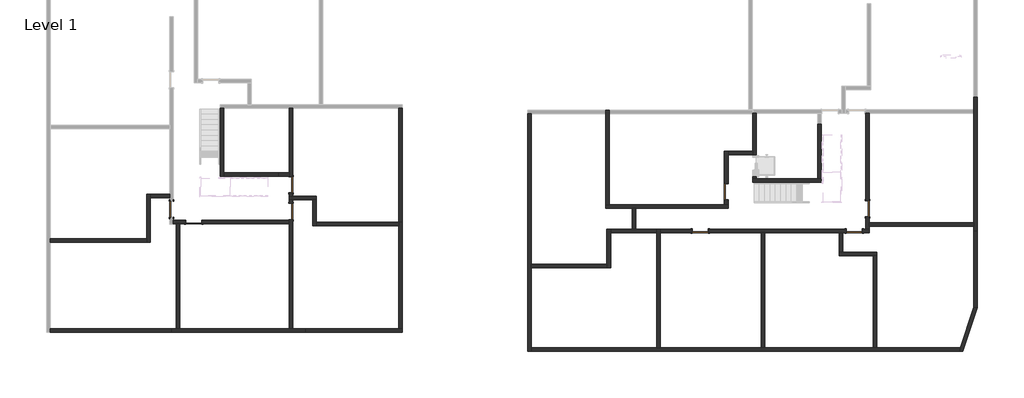
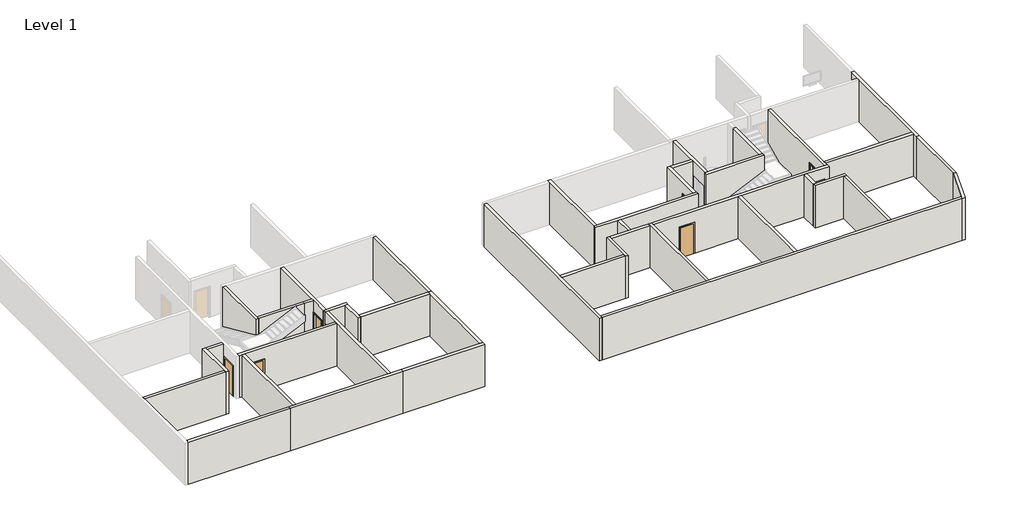
# One storey, part 1 of 2: 42 walls, 8 doors.
# Revit data of these elements (continued)
# Room, not placed, phase "New Construction", upper offset 0 cm, lower offset 0 cm
#   Number = "127"
#   Name = "Room"
# Room, not placed, phase "New Construction", upper offset 0 cm, lower offset 0 cm
#   Number = "128"
#   Name = "Room"
# Room, not placed, phase "New Construction", upper offset 0 cm, lower offset 0 cm
#   Number = "129"
#   Name = "Room"
# Room, not placed, phase "New Construction", upper offset 0 cm, lower offset 0 cm
#   Number = "91"
#   Name = "Room"
# Room at (-20321.225, 11202.195) mm, phase "New Construction", upper level "Level 1", upper offset 243.84 cm, lower offset 0 cm
#   Number = "130"
#   Name = "Room"
# Room at (-5594.466, -7580.79) mm, phase "New Construction", upper level "Level 1", upper offset 243.84 cm, lower offset 0 cm
#   Number = "131"
#   Name = "Room"
# Room at (-4954.966, -1430.614) mm, phase "New Construction", upper level "Level 1", upper offset 243.84 cm, lower offset 0 cm
#   Number = "132"
#   Name = "Room"
# Room at (-12237.947, 10302.814) mm, phase "New Construction", upper level "Level 1", upper offset 243.84 cm, lower offset 0 cm
#   Number = "133"
#   Name = "Room"
# Room, not placed, phase "New Construction", upper offset 0 cm, lower offset 0 cm
#   Number = ""
#   Name = ""
# Room, not placed, phase "New Construction", upper offset 0 cm, lower offset 0 cm
#   Number = "70"
#   Name = "Room"
# Room, not placed, phase "New Construction", upper offset 0 cm, lower offset 0 cm
#   Number = "71"
#   Name = "Room"
# Room, not placed, phase "New Construction", upper offset 0 cm, lower offset 0 cm
#   Number = "92"
#   Name = "Room"
# Room, not placed, phase "New Construction", upper offset 0 cm, lower offset 0 cm
#   Number = ""
#   Name = ""
# Room, not placed, phase "New Construction", upper offset 0 cm, lower offset 0 cm
#   Number = ""
#   Name = ""
# Room, not placed, phase "New Construction", upper offset 0 cm, lower offset 0 cm
#   Number = "37"
#   Name = "Room"
# Room, not placed, phase "New Construction", upper offset 0 cm, lower offset 0 cm
#   Number = ""
#   Name = "Banyo"
# Room, not placed, phase "New Construction", upper offset 0 cm, lower offset 0 cm
#   Number = ""
#   Name = ""
# Room, not placed, phase "New Construction", upper offset 0 cm, lower offset 0 cm
#   Number = ""
#   Name = "Yatak Odası"
# Room, not placed, phase "New Construction", upper offset 0 cm, lower offset 0 cm
#   Number = "39"
#   Name = "Room"
# Room, not placed, phase "New Construction", upper offset 0 cm, lower offset 0 cm
#   Number = ""
#   Name = "Salon-Mutfak"
# Area at (-11214.009, 13625.616) mm, upper offset 243.84 cm, lower offset 0 cm
#   Number = "9"
#   Name = "Area"
# Room, not placed, phase "New Construction", upper offset 0 cm, lower offset 0 cm
#   Number = "134"
#   Name = "Room"
# Room at (-19334.034, -2481.955) mm, phase "New Construction", upper level "Level 1", upper offset 243.84 cm, lower offset 0 cm
#   Number = "135"
#   Name = "Room"
# Room, not placed, phase "New Construction", upper offset 0 cm, lower offset 0 cm
#   Number = "40"
#   Name = "Room"
# Room, not placed, phase "New Construction", upper offset 0 cm, lower offset 0 cm
#   Number = "41"
#   Name = "Room"
# Area, not placed, upper offset 0 cm, lower offset 0 cm
#   Number = "8"
#   Name = "Dere Parsel Toplam Alan"
# Room, not placed, phase "New Construction", upper offset 0 cm, lower offset 0 cm
#   Number = "108"
#   Name = "ASANSÖR"
# Room, not placed, phase "New Construction", upper offset 0 cm, lower offset 0 cm
#   Number = "89"
#   Name = "Room"
# Room, not placed, phase "New Construction", upper offset 0 cm, lower offset 0 cm
#   Number = "19"
#   Name = "Room"
# Room, not placed, phase "New Construction", upper offset 0 cm, lower offset 0 cm
#   Number = ""
#   Name = ""
# Room, not placed, phase "New Construction", upper offset 0 cm, lower offset 0 cm
#   Number = "21"
#   Name = "Room"
# Room, not placed, phase "New Construction", upper offset 0 cm, lower offset 0 cm
#   Number = "22"
#   Name = "Room"
# Room, not placed, phase "New Construction", upper offset 0 cm, lower offset 0 cm
#   Number = "23"
#   Name = "Room"
# Room, not placed, phase "New Construction", upper offset 0 cm, lower offset 0 cm
#   Number = "24"
#   Name = "Room"
# Room, not placed, phase "New Construction", upper offset 0 cm, lower offset 0 cm
#   Number = "25"
#   Name = "Room"
# Room, not placed, phase "New Construction", upper offset 0 cm, lower offset 0 cm
#   Number = "64"
#   Name = "Room"
# Room, not placed, phase "New Construction", upper offset 0 cm, lower offset 0 cm
#   Number = "65"
#   Name = "Room"
# Room, not placed, phase "New Construction", upper offset 0 cm, lower offset 0 cm
#   Number = "66"
#   Name = "Room"
# Room, not placed, phase "New Construction", upper offset 0 cm, lower offset 0 cm
#   Number = ""
#   Name = ""
# Room, not placed, phase "New Construction", upper offset 0 cm, lower offset 0 cm
#   Number = "27"
#   Name = "Room"
# Room, not placed, phase "New Construction", upper offset 0 cm, lower offset 0 cm
#   Number = "42"
#   Name = "Room"
# Area, not placed, upper offset 0 cm, lower offset 0 cm
#   Number = "2"
#   Name = "Area"
# Room, not placed, phase "New Construction", upper offset 0 cm, lower offset 0 cm
#   Number = "43"
#   Name = "Room"
# Room, not placed, phase "New Construction", upper offset 0 cm, lower offset 0 cm
#   Number = ""
#   Name = ""
# Room, not placed, phase "New Construction", upper offset 0 cm, lower offset 0 cm
#   Number = "94"
#   Name = "Room"
# Room, not placed, phase "New Construction", upper offset 0 cm, lower offset 0 cm
#   Number = ""
#   Name = ""
# Room at (-18935.383, 3898.657) mm, phase "New Construction", upper level "Level 1", upper offset 243.84 cm, lower offset 0 cm
#   Number = "136"
#   Name = "Room"
# Room, not placed, phase "New Construction", upper offset 0 cm, lower offset 0 cm
#   Number = "1"
#   Name = "Room"
# Area, not placed, upper offset 0 cm, lower offset 0 cm
#   Number = "3"
#   Name = "Area"
# Room, not placed, phase "New Construction", upper offset 0 cm, lower offset 0 cm
#   Number = "7"
#   Name = "Room"
# Room, not placed, phase "New Construction", upper offset 0 cm, lower offset 0 cm
#   Number = "8"
#   Name = "Room"
# Room, not placed, phase "New Construction", upper offset 0 cm, lower offset 0 cm
#   Number = "2"
#   Name = "Room"
# Room, not placed, phase "New Construction", upper offset 0 cm, lower offset 0 cm
#   Number = "46"
#   Name = "Room"
# Room, not placed, phase "New Construction", upper offset 0 cm, lower offset 0 cm
#   Number = "3"
#   Name = "Room"
# Room, not placed, phase "New Construction", upper offset 0 cm, lower offset 0 cm
#   Number = ""
#   Name = ""
# Room, not placed, phase "New Construction", upper offset 0 cm, lower offset 0 cm
#   Number = "4"
#   Name = "Room"
# Area, not placed, upper offset 0 cm, lower offset 0 cm
#   Number = "1"
#   Name = "Area"
# Room, not placed, phase "New Construction", upper offset 0 cm, lower offset 0 cm
#   Number = ""
#   Name = ""
# Room, not placed, phase "New Construction", upper offset 0 cm, lower offset 0 cm
#   Number = "29"
#   Name = "Room"
# Area, not placed, upper offset 0 cm, lower offset 0 cm
#   Number = "7"
#   Name = "Dere Parsel Toplam Alan"
# Room, not placed, phase "New Construction", upper offset 0 cm, lower offset 0 cm
#   Number = "95"
#   Name = "ASANSÖR"
# Room, not placed, phase "New Construction", upper offset 0 cm, lower offset 0 cm
#   Number = "96"
#   Name = "Room"
# Room, not placed, phase "New Construction", upper offset 0 cm, lower offset 0 cm
#   Number = "97"
#   Name = "7"
# Room, not placed, phase "New Construction", upper offset 0 cm, lower offset 0 cm
#   Number = "98"
#   Name = "8"
# Room, not placed, phase "New Construction", upper offset 0 cm, lower offset 0 cm
#   Number = "99"
#   Name = "9"
# Room, not placed, phase "New Construction", upper offset 0 cm, lower offset 0 cm
#   Number = "100"
#   Name = "1"
# Room, not placed, phase "New Construction", upper offset 0 cm, lower offset 0 cm
#   Number = "101"
#   Name = "5"
# Room, not placed, phase "New Construction", upper offset 0 cm, lower offset 0 cm
#   Number = "102"
#   Name = "2"
# Room, not placed, phase "New Construction", upper offset 0 cm, lower offset 0 cm
#   Number = "103"
#   Name = "4"
# Room, not placed, phase "New Construction", upper offset 0 cm, lower offset 0 cm
#   Number = "104"
#   Name = "3"
# Room, not placed, phase "New Construction", upper offset 0 cm, lower offset 0 cm
#   Number = "105"
#   Name = "6"
